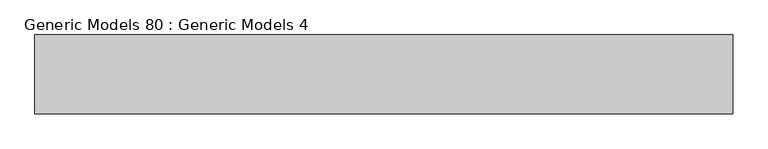
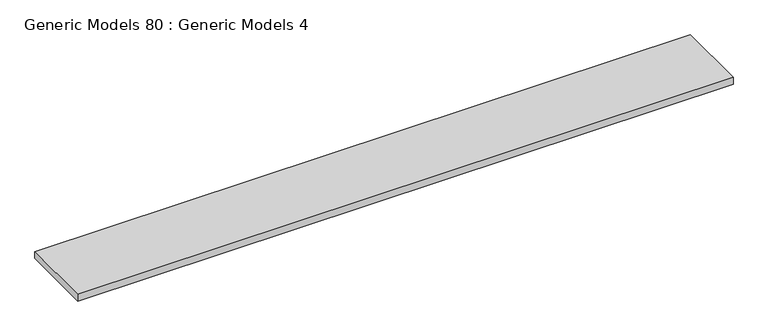
"""IFC4 building model written with IfcOpenShell, lengths in millimetres: proxy geometry, Generic Models 80 : Generic Models 4."""

from ifc_helpers import new_model, si_unit, frame, origin, place, context, project, spatial, polyline, outline, extrude, source, transform, mapped, element, save


def generic_models_80_generic_models_4_4eb52efd(model_context):
    return source(origin(), model_context, "Body", "SweptSolid", [
        extrude(outline(polyline([(27986.3863332, -7352.2318256), (27986.3863332, -7897.898997), (23168.0573109, -7897.898997), (23168.0573109, -7352.2318256), (27986.3863332, -7352.2318256)])), frame((0.0, 0.0, 123157.996), z_axis=(0.0, 0.0, 1.0), x_axis=(1.0, 0.0, 0.0)), (0.0, 0.0, 1.0), 50.8),
    ])


if __name__ == "__main__":
    model = new_model("IFC4")
    model_context = context("Model", 3, world=origin())
    ifc_project = project(units=[si_unit("LENGTHUNIT", "METRE", prefix="MILLI")], contexts=[model_context])
    site = spatial("IfcSite", under=ifc_project)
    building = spatial("IfcBuilding", under=site)
    placement = place(None, origin())
    generic_models_80_generic_models_4_shape = generic_models_80_generic_models_4_4eb52efd(model_context)
    element("IfcBuildingElementProxy", 1, Name="Generic Models 80 : Generic Models 4", ObjectType="Generic Models 80 : Generic Models 4", at=placement, inside=building, context=model_context, shape_type="MappedRepresentation", body=[
        mapped(generic_models_80_generic_models_4_shape, transform((0.0, 0.0, 0.0), x_axis=(1.0, 0.0, 0.0), y_axis=(0.0, 1.0, 0.0), z_axis=(0.0, 0.0, 1.0))),
    ])
    save(model, "model.ifc")

# Revit data of these elements
# Element 1 (IfcBuildingElementProxy, "Generic Models 80 : Generic Models 4")
#   Materials on its faces: "_2\" SAND"
# Materials
#   "_2\" SAND": class "Generic", colour RGB 245 226 173, transparency 0, Cost = 0
